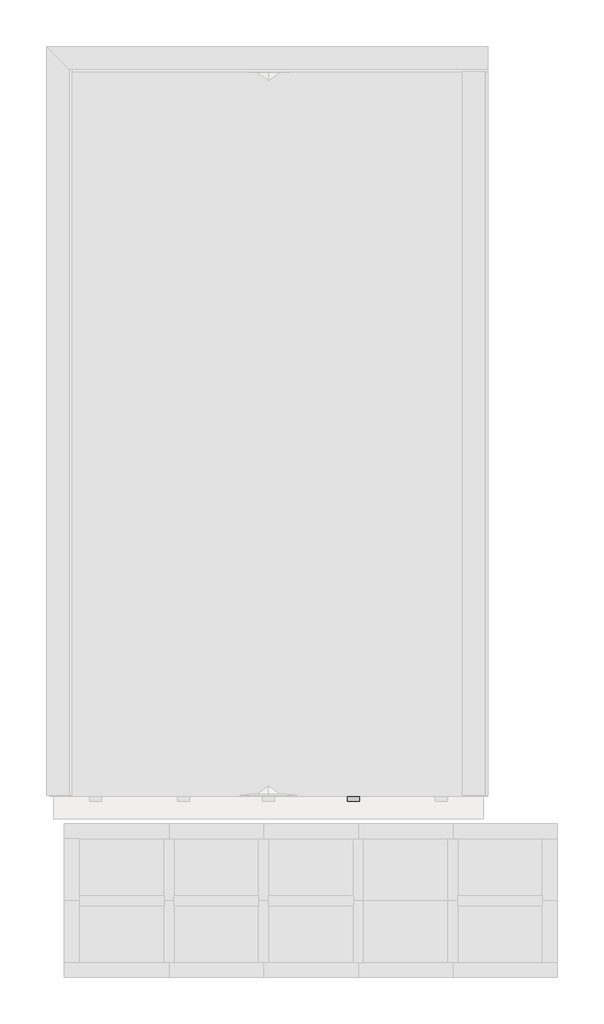
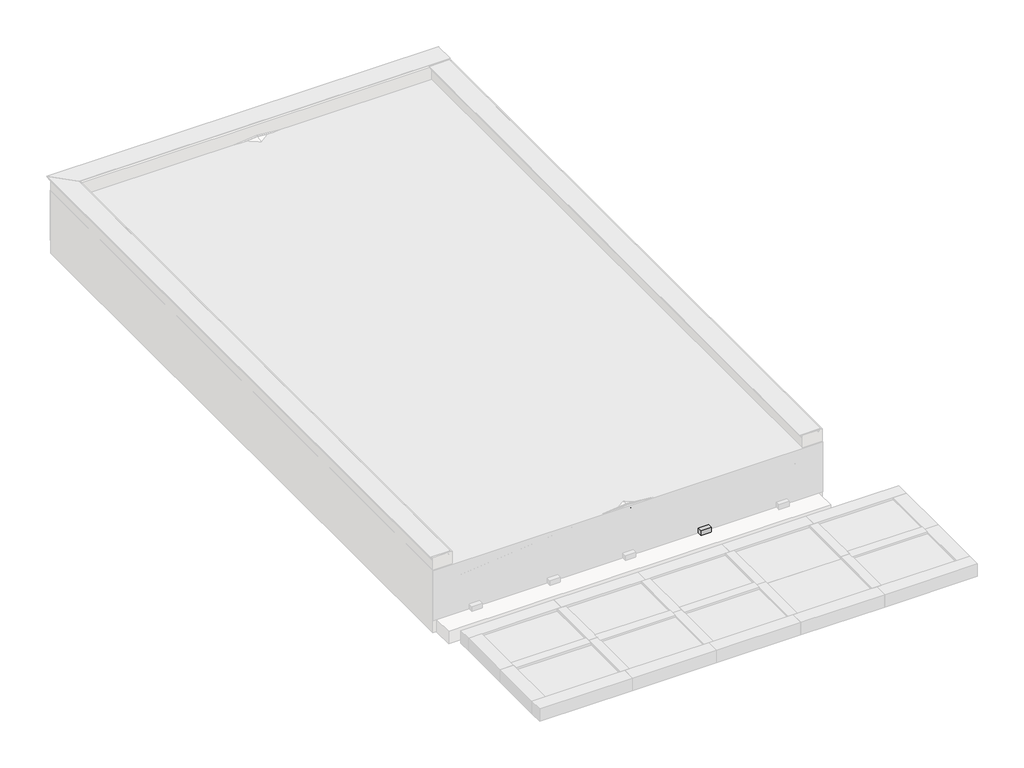
# One storey, part 2 of 3: 37 beams, 6 columns.
# Revit data of these elements (continued)
# Elements 1, 2, 3, 4, 6, 7 (IfcBeam, "Madeira de lei : Berço 6x12cm") (continued)
#   Phase Created = CC_AP
#   Materials on its faces: ".MADEIRAMENTO"
# Element 5 (IfcBeam, "Madeira de lei : Berço 6x12cm")
#   Comments = ""
#   Uso = "TELHADOS ESTRUTURAS"
#   Compr Cmcl = 7.00 m
#   Structural Material = .MADEIRAMENTO
#   Phase Created = CC_AP
#   Materials on its faces: ".MADEIRAMENTO"
# Element 8 (IfcBeam, "Cumeeira Telha Ondulada : Fibrocimento")
#   Comments = ""
#   Uso = "TELHADOS TELHAS"
#   Phase Created = CC_AP
#   Materials on its faces: ".TELHA DE FIBROCIMENTO"
# Elements 9, 10, 11, 12, 13, 14, 15, 16, 17, 18, 19, 20, 21, 22, 23, 24, 25, 26, 27, 28, 29, 30, 31, 32, 33, 34, 35, 36 (IfcBeam, "Telha Ondulada : Fibrocimento")
#   Uso = "TELHADOS TELHAS"
#   Phase Created = CC_AP
#   Materials on its faces: ".TELHA DE FIBROCIMENTO"
# Element 37 (IfcBeam, "Madeira de lei : Viga Cumeeira 6x16cm")
#   Comments = ""
#   Uso = "TELHADOS MADEIRAMENTO"
#   Compr Cmcl = 7.50 m
#   Structural Material = .MADEIRAMENTO
#   Phase Created = CC_AP
#   Materials on its faces: ".MADEIRAMENTO"
# Elements 38, 39, 40, 41, 42, 43 (IfcColumn, "Madeira de lei-Coluna : Pontalete 6X16cm")
#   Comments = ""
#   Uso = "TELHADOS ESTRUTURAS"
#   Compr Cmcl = 2.00 m
#   Structural Material = .MADEIRAMENTO
#   Phase Created = CC_AP
#   Materials on its faces: ".MADEIRAMENTO"
# Materials
#   ".TELHA DE FIBROCIMENTO": class "CC_TELHADO", colour RGB 77 77 76, transparency 0, Description = "TELHA ONDULADA FIBROCIMENTO", Cost = 0
#   ".MADEIRAMENTO": class ".CC_MADEIRAS", colour RGB 212 179 113, transparency 0, Cost = 0
# Room, not placed, phase "CC_AP", upper offset 0.00 m, lower offset 0.00 m
#   Number = "31"
#   Name = "Room"
# Room, not placed, phase "CC_AP", upper offset 0.00 m, lower offset 0.00 m
#   Number = "34"
#   Name = "Room"
